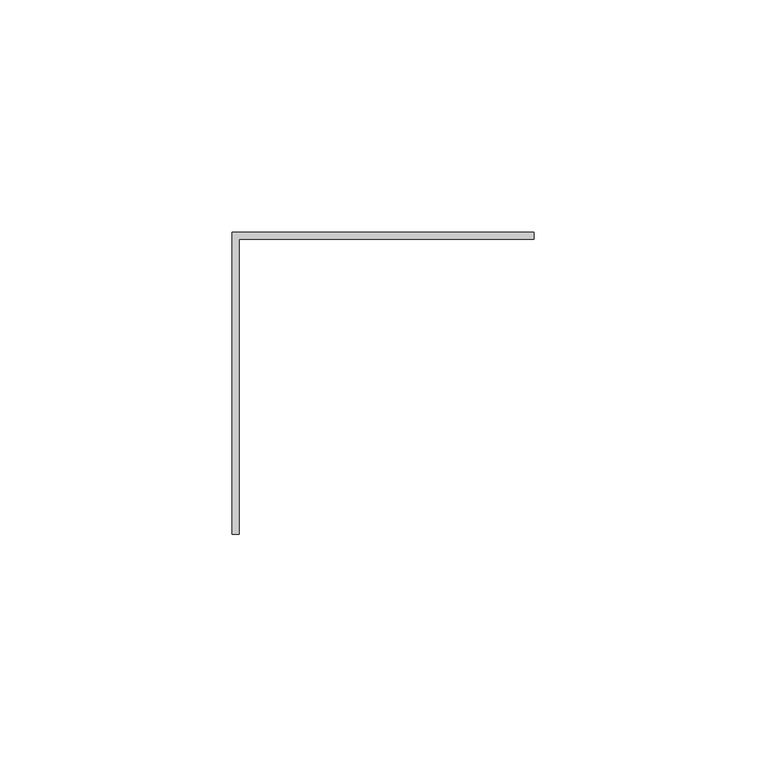
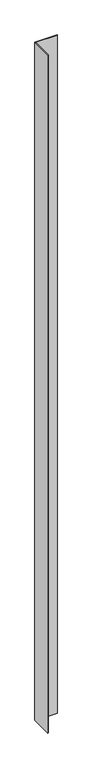
"""IFC4 building model written with IfcOpenShell, lengths in millimetres: proxy geometry, Generic Models 2:Generic Models 2:310765:Generic Models 2:310765 : Generic Models 2:Generic Models 2:310765:79 : Generic Models 2:Generic Models 2:310765:Generic Models 2:310765 : Generic Models 2:Generic Models 2:310765:300385."""

from ifc_helpers import new_model, si_unit, frame, origin, place, context, project, spatial, polyline, outline, extrude, source, transform, mapped, element, save


def generic_models_61527323(model_context):
    return source(origin(), model_context, "Body", "SweptSolid", [
        extrude(outline(polyline([(560410.9054739, -578791.1413841), (560347.4054739, -578791.1413841), (560347.4054739, -578854.6413841), (560345.8179739, -578854.6413841), (560345.8179739, -578789.5538841), (560410.9054739, -578789.5538841), (560410.9054739, -578791.1413841)])), frame((0.0, 0.0, 4033.8810286), z_axis=(0.0, 0.0, 1.0), x_axis=(1.0, 0.0, 0.0)), (0.0, 0.0, 1.0), 2100.2189714),
    ])


if __name__ == "__main__":
    model = new_model("IFC4")
    model_context = context("Model", 3, world=origin())
    ifc_project = project(units=[si_unit("LENGTHUNIT", "METRE", prefix="MILLI")], contexts=[model_context])
    site = spatial("IfcSite", under=ifc_project)
    building = spatial("IfcBuilding", under=site)
    placement = place(None, origin())
    generic_models_shape = generic_models_61527323(model_context)
    element("IfcBuildingElementProxy", 1, Name="Generic Models 2:Generic Models 2:310765:Generic Models 2:310765 : Generic Models 2:Generic Models 2:310765:79 : Generic Models 2:Generic Models 2:310765:Generic Models 2:310765 : Generic Models 2:Generic Models 2:310765:300385", ObjectType="Generic Models 2:Generic Models 2:310765:Generic Models 2:310765 : Generic Models 2:Generic Models 2:310765:79 : Generic Models 2:Generic Models 2:310765:Generic Models 2:310765 : Generic Models 2:Generic Models 2:310765:300385", at=placement, inside=building, context=model_context, shape_type="MappedRepresentation", body=[
        mapped(generic_models_shape, transform((0.0, 0.0, 0.0), x_axis=(1.0, 0.0, 0.0), y_axis=(0.0, 1.0, 0.0), z_axis=(0.0, 0.0, 1.0))),
    ])
    save(model, "model.ifc")

# Revit data of these elements
# Type "Generic Models 2:Generic Models 2:310765:Generic Models 2:310765 : Generic Models 2:Generic Models 2:310765:79 : Generic Models 2:Generic Models 2:310765:Generic Models 2:310765 : Generic Models 2:Generic Models 2:310765:300385"
#   NameOverride = "Generic Models 2:Generic Models 2:310765:Generic Models 2:310765 : Generic Models 2:Generic Models 2:310765:300385"
#   ObjectTypeOverride = "Generic Models 2:310765 : Generic Models 2:Generic Models 2:310765"
#   Reference = "Generic Models 2"
#   Tag = "300385"
# Element 1 (IfcBuildingElementProxy, "Generic Models 2:Generic Models 2:310765:Generic Models 2:310765 : Generic Models 2:Generic Models 2:310765:79 : Generic Models 2:Generic Models 2:310765:Generic Models 2:310765 : Generic Models 2:Generic Models 2:310765:300385")
#   Materials on its faces: "BRAKE METAL CLOSURE TRIM"
# Materials
#   "BRAKE METAL CLOSURE TRIM": class "Unassigned", colour RGB 182 182 182, transparency 0, Cost = 0
